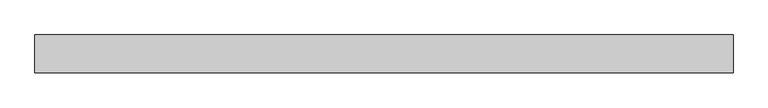
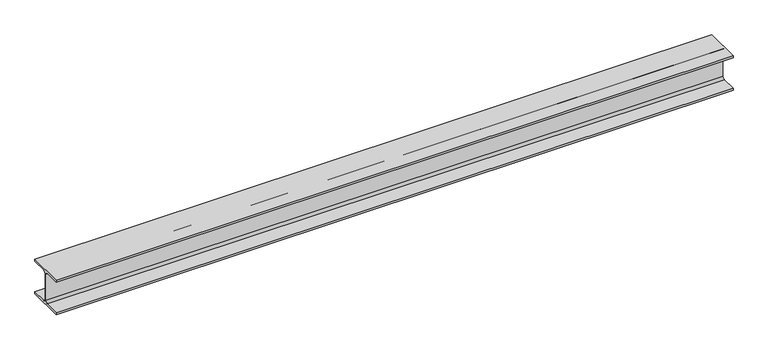
"""IFC4 building model written with IfcOpenShell, lengths in millimetres: beam geometry, 0912_Steel Framing_H-KSD3502 : H_SB_ASB_H-200x200x8x12."""

from ifc_helpers import new_model, si_unit, point, frame, frame_2d, origin, place, context, project, spatial, polyline, circle_curve, trimmed, segment, composite_curve, outline, extrude, source, transform, mapped, element, save


def beam_0fa2dae1(model_context):
    return source(origin(), model_context, "Body", "SweptSolid", [
        extrude(outline(composite_curve([segment(polyline([(100.0, -88.0), (100.0, -100.0), (-100.0, -100.0), (-100.0, -88.0), (-17.0, -88.0)]), True, "CONTINUOUS"), segment(trimmed(circle_curve(frame_2d((-17.0, -75.0)), 13.0), [point((-17.0, -88.0))], [point((-4.0, -75.0))], True, "CARTESIAN"), True, "CONTINUOUS"), segment(polyline([(-4.0, -75.0), (-4.0, 75.0)]), True, "CONTINUOUS"), segment(trimmed(circle_curve(frame_2d((-17.0, 75.0)), 13.0), [point((-4.0, 75.0))], [point((-17.0, 88.0))], True, "CARTESIAN"), True, "CONTINUOUS"), segment(polyline([(-17.0, 88.0), (-100.0, 88.0), (-100.0, 100.0), (100.0, 100.0), (100.0, 88.0), (17.0, 88.0)]), True, "CONTINUOUS"), segment(trimmed(circle_curve(frame_2d((17.0, 75.0)), 13.0), [point((17.0, 88.0))], [point((4.0, 75.0))], True, "CARTESIAN"), True, "CONTINUOUS"), segment(polyline([(4.0, 75.0), (4.0, -75.0)]), True, "CONTINUOUS"), segment(trimmed(circle_curve(frame_2d((17.0, -75.0)), 13.0), [point((4.0, -75.0))], [point((17.0, -88.0))], True, "CARTESIAN"), True, "CONTINUOUS"), segment(polyline([(17.0, -88.0), (100.0, -88.0)]), True, "CONTINUOUS")], self_intersect=False)), frame((-1814.9907357, 0.0, 0.0), z_axis=(1.0, 0.0, 0.0), x_axis=(0.0, 1.0, 0.0)), (0.0, 0.0, 1.0), 3702.1907618),
    ])


if __name__ == "__main__":
    model = new_model("IFC4")
    model_context = context("Model", 3, world=origin())
    ifc_project = project(units=[si_unit("LENGTHUNIT", "METRE", prefix="MILLI")], contexts=[model_context])
    site = spatial("IfcSite", under=ifc_project)
    building = spatial("IfcBuilding", under=site)
    placement = place(None, origin())
    beam_shape = beam_0fa2dae1(model_context)
    element("IfcBeam", 1, ObjectType="0912_Steel Framing_H-KSD3502 : H_SB_ASB_H-200x200x8x12", at=placement, inside=building, context=model_context, shape_type="MappedRepresentation", body=[
        mapped(beam_shape, transform((0.0, 0.0, 0.0), x_axis=(1.0, 0.0, 0.0), y_axis=(0.0, 1.0, 0.0), z_axis=(0.0, 0.0, 1.0))),
    ])
    save(model, "model.ifc")

# Revit data of these elements
# Type "0912_Steel Framing_H-KSD3502 : H_SB_ASB_H-200x200x8x12"
#   H_WM Code_1 = "S01AA002-00001 | Main Steel Structure Fabrication Work | Shelter/Building | Medium Steel - Standard (90KG/M>Weight≥30KG/M) | Material: (   )"
#   H_WM Code_2 = "S03AA028-00001 | Main Steel Structure Erection Work | Shelter/Building | Medium Steel (90KG/M>Weight≥30KG/M) | Material: (   )"
#   H_WM Code_3 = "S01AA010-00001 | Main Steel Structure Fabrication Work | Shelter/Building | Steel Painting/Coating | for Non-Fireproofed Steel Surface, Surface Preparation, Primer, Second & Final Coat | Material: (   )"
#   H_Q'ty Cal Type Tag = "SB-Q2"
#   Width = 20.0 cm
#   Web Thickness = 0.8 cm
#   Web Fillet = 1.3 cm
#   Warping Constant = 141000.0 cm⁶
#   W = 0
#   Torsional Moment of Inertia = 26.2485 cm⁴
#   Section Area = 63.53 cm²
#   Plastic Modulus weak axis = 244.0 cm³
#   Plastic Modulus strong axis = 525.0 cm³
#   Perimeter = 1.16 m²/m
#   Nominal Weight = 49.90 kgf/m
#   Moment of Inertia weak axis = 1600.00 cm⁴
#   Moment of Inertia strong axis = 4720.00 cm⁴
#   Height = 20.0 cm
#   Flange Thickness = 1.2 cm
#   Elastic Modulus weak axis = 160.0 cm³
#   Elastic Modulus strong axis = 472.0 cm³
#   Centroid Vertical = 10.0 cm
#   Centroid Horizontal = 10.0 cm
#   Ix = 47200000
#   Length [instance default] = 1.5240 m
#   Zx = 525000
#   b = 0.2000 m
#   h = 0.2000 m
#   r = 0.0130 m
#   s = 0.0080 m
#   t = 0.0120 m
#   A = 0.006353 m²
#   Structural Material [instance default] = Steel, 45-345
#   Assembly Code = ""
# Element 1 (IfcBeam, "0912_Steel Framing_H-KSD3502 : H_SB_ASB_H-200x200x8x12")
#   Structural Material = none
# Materials
#   "Steel, 45-345": class "Metal", colour RGB 189 187 185, transparency 0, Description = "Steel 345 MPa", Cost = 0
